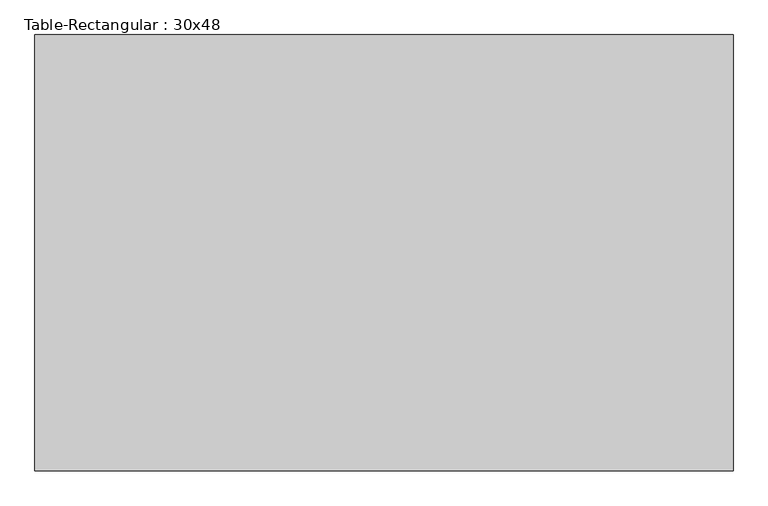
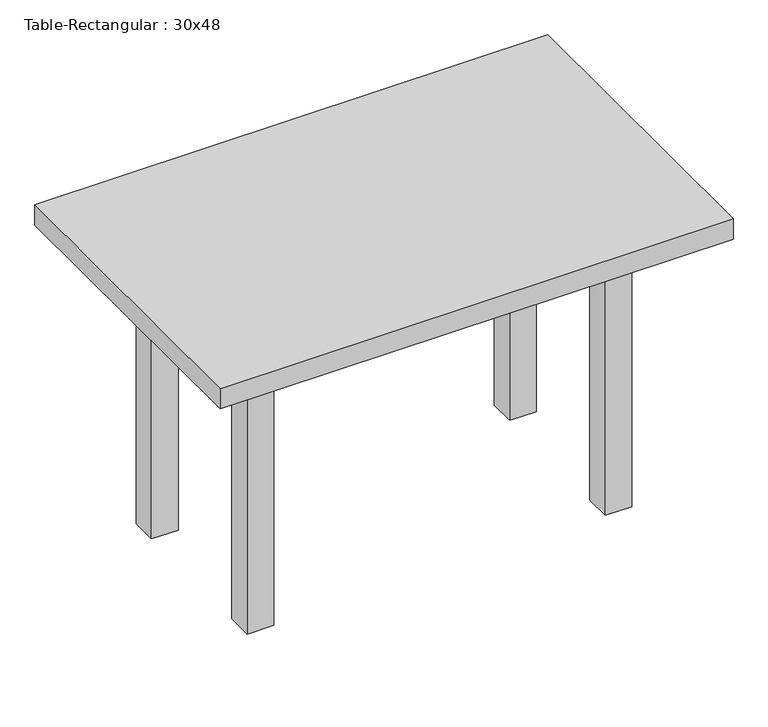
"""IFC4 building model written with IfcOpenShell, lengths in millimetres: furniture geometry, Table-Rectangular : 30x48."""

from ifc_helpers import new_model, si_unit, frame, origin, origin_with_axes, place, context, project, spatial, polyline, outline, extrude, source, transform, mapped, element, save


def table_rectangular_30x48_cda8806a(model_context):
    return source(origin(), model_context, "Body", "SweptSolid", [
        extrude(outline(polyline([(393.7, 190.5), (393.7, 165.1), (-393.7, 165.1), (-393.7, 190.5), (393.7, 190.5)])), frame((0.0, 0.0, 609.6), z_axis=(0.0, 0.0, 1.0), x_axis=(1.0, 0.0, 0.0)), (0.0, 0.0, 1.0), 101.6),
        extrude(outline(polyline([(393.7, -190.5), (-393.7, -190.5), (-393.7, -165.1), (393.7, -165.1), (393.7, -190.5)])), frame((0.0, 0.0, 609.6), z_axis=(0.0, 0.0, 1.0), x_axis=(1.0, 0.0, 0.0)), (0.0, 0.0, 1.0), 101.6),
        extrude(outline(polyline([(-406.4, -165.1), (-431.8, -165.1), (-431.8, 165.1), (-406.4, 165.1), (-406.4, -165.1)])), frame((0.0, 0.0, 609.6), z_axis=(0.0, 0.0, 1.0), x_axis=(1.0, 0.0, 0.0)), (0.0, 0.0, 1.0), 101.6),
        extrude(outline(polyline([(406.4, -165.1), (406.4, 165.1), (431.8, 165.1), (431.8, -165.1), (406.4, -165.1)])), frame((0.0, 0.0, 609.6), z_axis=(0.0, 0.0, 1.0), x_axis=(1.0, 0.0, 0.0)), (0.0, 0.0, 1.0), 101.6),
        extrude(outline(polyline([(-393.7, 228.6), (-393.7, 165.1), (-457.2, 165.1), (-457.2, 228.6), (-393.7, 228.6)])), origin_with_axes(), (0.0, 0.0, 1.0), 711.2),
        extrude(outline(polyline([(393.7, 228.6), (457.2, 228.6), (457.2, 165.1), (393.7, 165.1), (393.7, 228.6)])), origin_with_axes(), (0.0, 0.0, 1.0), 711.2),
        extrude(outline(polyline([(-393.7, -228.6), (-457.2, -228.6), (-457.2, -165.1), (-393.7, -165.1), (-393.7, -228.6)])), origin_with_axes(), (0.0, 0.0, 1.0), 711.2),
        extrude(outline(polyline([(393.7, -228.6), (393.7, -165.1), (457.2, -165.1), (457.2, -228.6), (393.7, -228.6)])), origin_with_axes(), (0.0, 0.0, 1.0), 711.2),
        extrude(outline(polyline([(609.6, 381.0), (609.6, -381.0), (-609.6, -381.0), (-609.6, 381.0), (609.6, 381.0)])), frame((0.0, 0.0, 711.2), z_axis=(0.0, 0.0, 1.0), x_axis=(1.0, 0.0, 0.0)), (0.0, 0.0, 1.0), 50.8),
    ])


if __name__ == "__main__":
    model = new_model("IFC4")
    model_context = context("Model", 3, world=origin())
    ifc_project = project(units=[si_unit("LENGTHUNIT", "METRE", prefix="MILLI")], contexts=[model_context])
    site = spatial("IfcSite", under=ifc_project)
    building = spatial("IfcBuilding", under=site)
    placement = place(None, origin())
    table_rectangular_30x48_shape = table_rectangular_30x48_cda8806a(model_context)
    element("IfcFurniture", 1, ObjectType="Table-Rectangular : 30x48", at=placement, inside=building, context=model_context, shape_type="MappedRepresentation", body=[
        mapped(table_rectangular_30x48_shape, transform((0.0, 0.0, 0.0), x_axis=(1.0, 0.0, 0.0), y_axis=(0.0, 1.0, 0.0), z_axis=(0.0, 0.0, 1.0))),
    ])
    save(model, "model.ifc")

# Revit data of these elements
# Type "Table-Rectangular : 30x48"
#   Assembly Code = "E2020200"
#   Height = 2' - 6"
#   Length = 4' - 0"
#   Width = 2' - 6"
#   Base Material = Birch
#   Top Material = Birch
# Element 1 (IfcFurniture, "Table-Rectangular : 30x48")
#   Materials on its faces: "Birch"
# Materials
#   "Birch": class "Wood", colour RGB 255 255 255, transparency 0, Description = "Betula Alleghaniensis", Cost = 0
